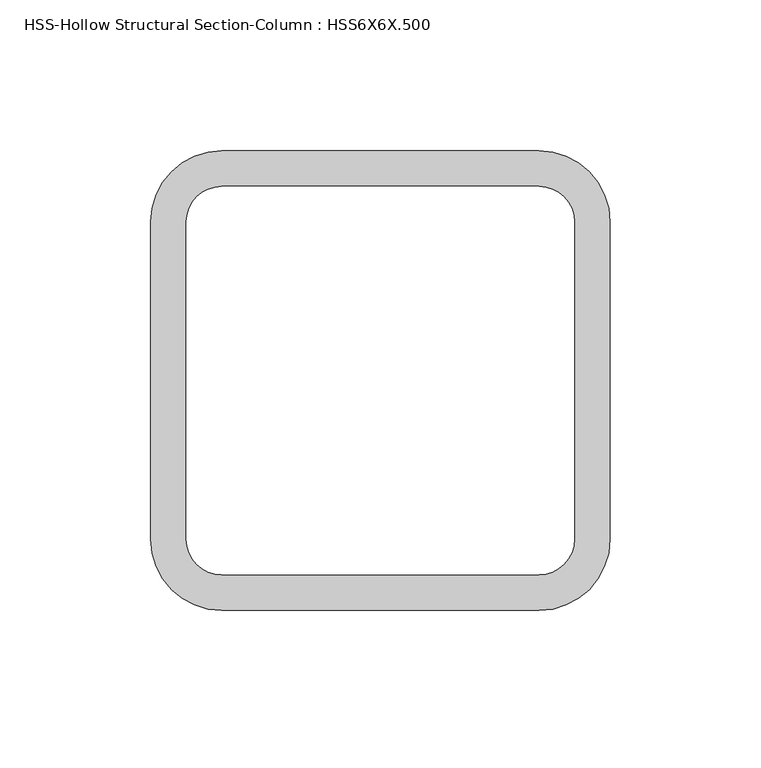
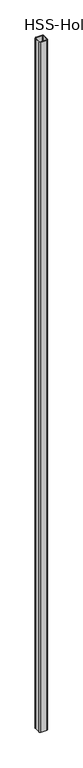
"""IFC4 building model written with IfcOpenShell, lengths in millimetres: column geometry, HSS-Hollow Structural Section-Column : HSS6X6X.500."""

import ifcopenshell
import ifcopenshell.guid

model = None  # the IFC model being written
_history = None  # IfcOwnerHistory: only IFC2X3 demands one
_inside = {}  # id of a spatial element -> (the spatial element, [elements in it])
_under = {}  # id of a project, library or spatial element -> (it, [spatial elements below it])
_declared = {}  # id of a project -> (the project, [libraries it declares])
_typed = {}  # id of a type object -> (the type object, [elements of that type])
_made_of = {}  # id of a material, layer set ... -> (it, [elements and type objects made of it])


def new_model(schema):
    """Start an empty IFC model of exactly this schema.

    Asked for "IFC4X3", IfcOpenShell would pick the latest addendum, in which some entities
    have other attributes; the version numbers below select the first issue.
    IFC2X3 requires an IfcOwnerHistory on every rooted entity: one is made here for all.
    """
    global model, _history
    if schema == "IFC4X3":
        model = ifcopenshell.file(schema_version=(4, 3, 0, 0))
    else:
        model = ifcopenshell.file(schema=schema)
    _inside.clear()
    _under.clear()
    _declared.clear()
    _typed.clear()
    _made_of.clear()
    _history = None
    if model.schema == "IFC2X3":
        org = make("IfcOrganization", Name="unknown")
        user = make(
            "IfcPersonAndOrganization",
            ThePerson=make("IfcPerson", FamilyName="unknown"),
            TheOrganization=org,
        )
        app = make(
            "IfcApplication",
            ApplicationDeveloper=org,
            Version="unknown",
            ApplicationFullName="unknown",
            ApplicationIdentifier="unknown",
        )
        _history = make(
            "IfcOwnerHistory",
            OwningUser=user,
            OwningApplication=app,
            ChangeAction="ADDED",
            CreationDate=0,
        )
    return model


def make(cls, **values):
    """One entity of the class cls with the attributes given. An attribute that is None is left unset."""
    return model.create_entity(
        cls, **{name: value for name, value in values.items() if value is not None}
    )


def rooted(cls, **values):
    """An entity with a GlobalId (a new one), such as an element, a storey or a relation."""
    return make(cls, GlobalId=ifcopenshell.guid.new(), OwnerHistory=_history, **values)


def si_unit(unit_type, name, prefix=None):
    """IfcSIUnit, for example si_unit("LENGTHUNIT", "METRE", prefix="MILLI")."""
    return make("IfcSIUnit", UnitType=unit_type, Prefix=prefix, Name=name)


def assignment(units):
    """IfcUnitAssignment: the units of a project."""
    return None if units is None else make("IfcUnitAssignment", Units=units)


def point(xyz):
    """IfcCartesianPoint."""
    return None if xyz is None else make("IfcCartesianPoint", Coordinates=xyz)


def direction(xyz):
    """IfcDirection."""
    return None if xyz is None else make("IfcDirection", DirectionRatios=xyz)


def frame(location, z_axis=None, x_axis=None):
    """IfcAxis2Placement3D, a coordinate frame: its origin and axes. An axis left out is left unset."""
    return make(
        "IfcAxis2Placement3D",
        Location=point(location),
        Axis=direction(z_axis),
        RefDirection=direction(x_axis),
    )


def frame_2d(location, x_axis=None):
    """IfcAxis2Placement2D, a coordinate frame in the plane: its origin and x axis."""
    return make(
        "IfcAxis2Placement2D", Location=point(location), RefDirection=direction(x_axis)
    )


def origin():
    """The frame at (0, 0, 0) with its axes left unset."""
    return frame((0.0, 0.0, 0.0))


def place(relative_to, where):
    """IfcLocalPlacement: puts the frame where relative to a parent placement (None: the world)."""
    return make(
        "IfcLocalPlacement", PlacementRelTo=relative_to, RelativePlacement=where
    )


def context(
    kind, dimensions, precision=None, world=None, true_north=None, identifier=None
):
    """IfcGeometricRepresentationContext, for example the 3D "Model" context."""
    return make(
        "IfcGeometricRepresentationContext",
        ContextIdentifier=identifier,
        ContextType=kind,
        CoordinateSpaceDimension=dimensions,
        Precision=precision,
        WorldCoordinateSystem=world,
        TrueNorth=true_north,
    )


def project(units=None, contexts=None):
    """IfcProject with its units and contexts."""
    return rooted(
        "IfcProject",
        Name="project",
        RepresentationContexts=contexts,
        UnitsInContext=assignment(units),
    )


def spatial(cls, under=None, at=None, **own):
    """A site, building, storey or space (cls), placed at a placement, below another one or the project."""
    s = rooted(cls, ObjectPlacement=at, **own)
    if under is not None:
        _under.setdefault(under.id(), (under, []))[1].append(s)
    return s


def polyline(points):
    """IfcPolyline through the points."""
    return make("IfcPolyline", Points=[point(p) for p in points])


def circle_curve(where, radius):
    """IfcCircle in the frame where."""
    return make("IfcCircle", Position=where, Radius=radius)


def trimmed(basis, trim1, trim2, sense, master):
    """IfcTrimmedCurve: the piece of a basis curve between two trims."""
    return make(
        "IfcTrimmedCurve",
        BasisCurve=basis,
        Trim1=trim1,
        Trim2=trim2,
        SenseAgreement=sense,
        MasterRepresentation=master,
    )


def segment(curve, same_sense, transition):
    """IfcCompositeCurveSegment."""
    return make(
        "IfcCompositeCurveSegment",
        Transition=transition,
        SameSense=same_sense,
        ParentCurve=curve,
    )


def composite_curve(segments, self_intersect=None):
    """IfcCompositeCurve: segments joined end to end."""
    return make("IfcCompositeCurve", Segments=segments, SelfIntersect=self_intersect)


def outline(outer, holes=None, kind="AREA"):
    """IfcArbitraryClosedProfileDef: a profile drawn as a closed curve; with holes, ...WithVoids."""
    if holes is None:
        return make("IfcArbitraryClosedProfileDef", ProfileType=kind, OuterCurve=outer)
    return make(
        "IfcArbitraryProfileDefWithVoids",
        ProfileType=kind,
        OuterCurve=outer,
        InnerCurves=holes,
    )


def extrude(swept, where, along, depth):
    """IfcExtrudedAreaSolid: the profile swept, set in the frame where, extruded along a direction by depth."""
    return make(
        "IfcExtrudedAreaSolid",
        SweptArea=swept,
        Position=where,
        ExtrudedDirection=direction(along),
        Depth=depth,
    )


def shape(context_of_items, identifier, shape_type, items):
    """IfcShapeRepresentation: the items that make up one representation, for example the "Body"."""
    return make(
        "IfcShapeRepresentation",
        ContextOfItems=context_of_items,
        RepresentationIdentifier=identifier,
        RepresentationType=shape_type,
        Items=items,
    )


def source(mapping_origin, context_of_items, identifier, shape_type, items):
    """IfcRepresentationMap: a shape defined once, which mapped items show again and again."""
    return make(
        "IfcRepresentationMap",
        MappingOrigin=mapping_origin,
        MappedRepresentation=shape(context_of_items, identifier, shape_type, items),
    )


def transform(
    local_origin,
    x_axis=None,
    y_axis=None,
    z_axis=None,
    scale=None,
    scale2=None,
    scale3=None,
    uniform=True,
):
    """IfcCartesianTransformationOperator3D, or its non-uniform kind. x_axis, y_axis, z_axis: its Axis1, 2, 3."""
    if uniform:
        return make(
            "IfcCartesianTransformationOperator3D",
            Axis1=direction(x_axis),
            Axis2=direction(y_axis),
            LocalOrigin=point(local_origin),
            Scale=scale,
            Axis3=direction(z_axis),
        )
    return make(
        "IfcCartesianTransformationOperator3DnonUniform",
        Axis1=direction(x_axis),
        Axis2=direction(y_axis),
        LocalOrigin=point(local_origin),
        Scale=scale,
        Axis3=direction(z_axis),
        Scale2=scale2,
        Scale3=scale3,
    )


def mapped(mapping_source, mapping_target):
    """IfcMappedItem: shows the shape of a source again, moved by a transform."""
    return make(
        "IfcMappedItem", MappingSource=mapping_source, MappingTarget=mapping_target
    )


def made_of(thing, what):
    """Note that an element or type object is made of a material, layer set ...; save() writes the relation."""
    if what is not None:
        _made_of.setdefault(what.id(), (what, []))[1].append(thing)
    return thing


def element(
    cls,
    number,
    at=None,
    inside=None,
    cuts=None,
    type_object=None,
    material=None,
    context=None,
    identifier="Body",
    shape_type=None,
    held_by="IfcProductDefinitionShape",
    body=None,
    shapes=None,
    **own,
):
    """One element of the class cls, such as IfcWall. Its Tag is "e" and its number.

    at: its placement. inside: the storey or other place that contains it. cuts: it is an
    opening in that element (IfcRelVoidsElement). A single representation is given by context,
    identifier, shape_type and body (its items); several are given by shapes. held_by: the class
    of the entity that holds the representations. save() writes the other relations.
    """
    e = rooted(cls, Tag="e%d" % number, ObjectPlacement=at, **own)
    if body is not None:
        shapes = [shape(context, identifier, shape_type, body)]
    if shapes is not None:
        e.Representation = make(held_by, Representations=shapes)
    if inside is not None:
        _inside.setdefault(inside.id(), (inside, []))[1].append(e)
    if cuts is not None:
        rooted(
            "IfcRelVoidsElement", RelatingBuildingElement=cuts, RelatedOpeningElement=e
        )
    if type_object is not None:
        _typed.setdefault(type_object.id(), (type_object, []))[1].append(e)
    return made_of(e, material)


def aggregate(whole, parts):
    """IfcRelAggregates: a whole, such as a stair, and the parts it consists of."""
    return rooted("IfcRelAggregates", RelatingObject=whole, RelatedObjects=parts)


def save(model, path):
    """Write the relations noted so far, then the file.

    IfcRelAggregates (storeys below a building ...), IfcRelContainedInSpatialStructure (elements
    in a storey), IfcRelDefinesByType, IfcRelAssociatesMaterial and IfcRelDeclares: one each for
    every whole, place, type object, material and project.
    """
    for whole, parts in _under.values():
        aggregate(whole, parts)
    for where, things in _inside.values():
        rooted(
            "IfcRelContainedInSpatialStructure",
            RelatedElements=things,
            RelatingStructure=where,
        )
    for kind, things in _typed.values():
        rooted("IfcRelDefinesByType", RelatedObjects=things, RelatingType=kind)
    for what, things in _made_of.values():
        rooted("IfcRelAssociatesMaterial", RelatedObjects=things, RelatingMaterial=what)
    for by, libraries in _declared.values():
        rooted("IfcRelDeclares", RelatingContext=by, RelatedDefinitions=libraries)
    model.write(path)


def hss_hollow_structural_section_column_hss6x6x_500_3a2aca85(model_context):
    return source(origin(), model_context, "Body", "SweptSolid", [
        extrude(outline(composite_curve([segment(trimmed(circle_curve(frame_2d((52.5859375, 52.5859375)), 23.6140625), [point((52.5859375, 76.2))], [point((76.2, 52.5859375))], False, "CARTESIAN"), True, "CONTINUOUS"), segment(polyline([(76.2, 52.5859375), (76.2, -52.5859375)]), True, "CONTINUOUS"), segment(trimmed(circle_curve(frame_2d((52.5859375, -52.5859375)), 23.6140625), [point((76.2, -52.5859375))], [point((52.5859375, -76.2))], False, "CARTESIAN"), True, "CONTINUOUS"), segment(polyline([(52.5859375, -76.2), (-52.5859375, -76.2)]), True, "CONTINUOUS"), segment(trimmed(circle_curve(frame_2d((-52.5859375, -52.5859375)), 23.6140625), [point((-52.5859375, -76.2))], [point((-76.2, -52.5859375))], False, "CARTESIAN"), True, "CONTINUOUS"), segment(polyline([(-76.2, -52.5859375), (-76.2, 52.5859375)]), True, "CONTINUOUS"), segment(trimmed(circle_curve(frame_2d((-52.5859375, 52.5859375)), 23.6140625), [point((-76.2, 52.5859375))], [point((-52.5859375, 76.2))], False, "CARTESIAN"), True, "CONTINUOUS"), segment(polyline([(-52.5859375, 76.2), (52.5859375, 76.2)]), True, "CONTINUOUS")], self_intersect=False), holes=[composite_curve([segment(polyline([(52.5859375, 64.3929688), (-52.5859375, 64.3929688)]), True, "CONTINUOUS"), segment(trimmed(circle_curve(frame_2d((-52.5859375, 52.5859375)), 11.8070313), [point((-52.5859375, 64.3929688))], [point((-64.3929688, 52.5859375))], True, "CARTESIAN"), True, "CONTINUOUS"), segment(polyline([(-64.3929688, 52.5859375), (-64.3929688, -52.5859375)]), True, "CONTINUOUS"), segment(trimmed(circle_curve(frame_2d((-52.5859375, -52.5859375)), 11.8070313), [point((-64.3929688, -52.5859375))], [point((-52.5859375, -64.3929687))], True, "CARTESIAN"), True, "CONTINUOUS"), segment(polyline([(-52.5859375, -64.3929687), (52.5859375, -64.3929687)]), True, "CONTINUOUS"), segment(trimmed(circle_curve(frame_2d((52.5859375, -52.5859375)), 11.8070312), [point((52.5859375, -64.3929687))], [point((64.3929687, -52.5859375))], True, "CARTESIAN"), True, "CONTINUOUS"), segment(polyline([(64.3929687, -52.5859375), (64.3929687, 52.5859375)]), True, "CONTINUOUS"), segment(trimmed(circle_curve(frame_2d((52.5859375, 52.5859375)), 11.8070312), [point((64.3929687, 52.5859375))], [point((52.5859375, 64.3929688))], True, "CARTESIAN"), True, "CONTINUOUS")], self_intersect=False)]), frame((0.0, 0.0, -609.6), z_axis=(0.0, 0.0, 1.0), x_axis=(1.0, 0.0, 0.0)), (0.0, 0.0, 1.0), 13004.8),
    ])


if __name__ == "__main__":
    model = new_model("IFC4")
    model_context = context("Model", 3, world=origin())
    ifc_project = project(units=[si_unit("LENGTHUNIT", "METRE", prefix="MILLI")], contexts=[model_context])
    site = spatial("IfcSite", under=ifc_project)
    building = spatial("IfcBuilding", under=site)
    placement = place(None, origin())
    hss_hollow_structural_section_column_hss6x6x_500_shape = hss_hollow_structural_section_column_hss6x6x_500_3a2aca85(model_context)
    element("IfcColumn", 1, ObjectType="HSS-Hollow Structural Section-Column : HSS6X6X.500", at=placement, inside=building, context=model_context, shape_type="MappedRepresentation", body=[
        mapped(hss_hollow_structural_section_column_hss6x6x_500_shape, transform((0.0, 0.0, 0.0), x_axis=(1.0, 0.0, 0.0), y_axis=(0.0, 1.0, 0.0), z_axis=(0.0, 0.0, 1.0))),
    ])
    save(model, "model.ifc")

# Revit data of these elements
# Type "HSS-Hollow Structural Section-Column : HSS6X6X.500"
#   Assembly Code = "B10"
#   Shape = "Square"
#   W = 35.1
#   Ht = 0' - 6"
#   b = 0' - 6"
#   kr = 0' - 0 119/128"
#   t = 0' - 0 119/256"
#   A = 0.07 SF
#   Structural Material [instance default] = Steel ASTM A500, Grade B, Rectangular and Square
# Element 1 (IfcColumn, "HSS-Hollow Structural Section-Column : HSS6X6X.500")
#   Materials on its faces: "Steel ASTM A500, Grade B, Rectangular and Square"
# Materials
#   "Steel ASTM A500, Grade B, Rectangular and Square": class "Metal", colour RGB 199 199 199, transparency 0, Description = "Carbon steel", Cost = 0
